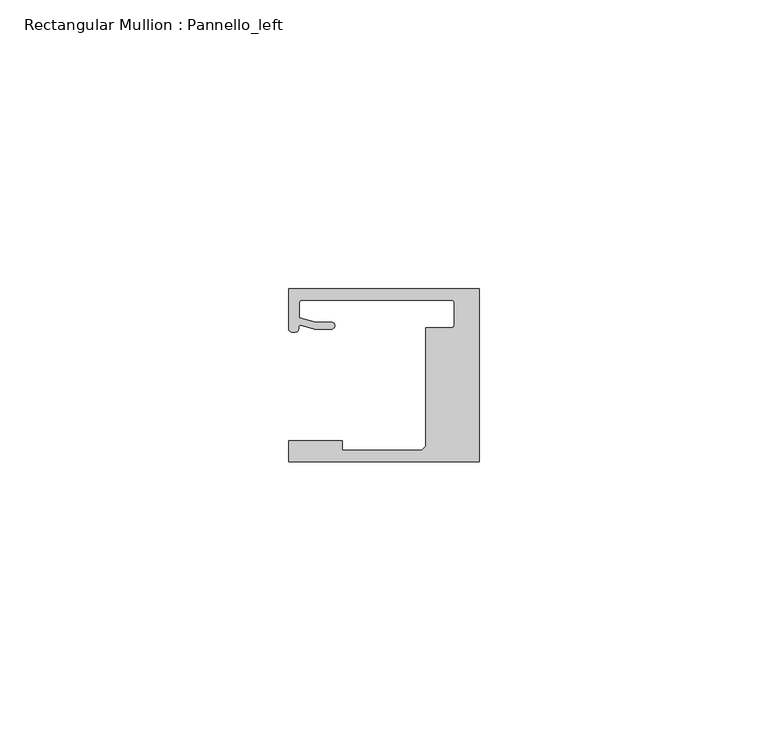
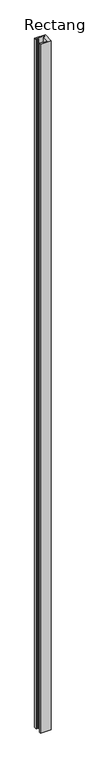
"""IFC4 building model written with IfcOpenShell, lengths in millimetres: member geometry, Rectangular Mullion : Pannello_left."""

from ifc_helpers import new_model, si_unit, frame, origin, place, context, project, spatial, polyline, circle_curve, source, transform, mapped, element, save
from ifc_brep_helpers import plane_surface, cylinder_surface, revolved_surface, extruded_surface, spline_curve, advanced_brep


def rectangular_mullion_pannello_left_b202d7d7(model_context):
    return source(origin(), model_context, "Body", "AdvancedBrep", [
        advanced_brep(
        [(-33.0, -15.0, 0.0), (0.0, -15.0, 0.0), (0.0, 15.0, 0.0), (-33.0000135, 15.0, 0.0), (-33.0000135, 8.0000472, 0.0), (-30.9223017, 8.6490241, 0.0), (-28.4999305, 7.9999523, 0.0), (-25.59998, 7.9999523, 0.0), (-25.59998, 9.1999523, 0.0), (-28.3419477, 9.1999523, 0.0), (-31.19998, 9.9657591, 0.0), (-31.19998, 12.50001, 0.0), (-30.69998, 13.00001, 0.0), (-4.7999726, 13.00001, 0.0), (-4.2999726, 12.50001, 0.0), (-4.2999726, 8.7500595, 0.0), (-4.7999726, 8.2500595, 0.0), (-9.2999726, 8.2500595, 0.0), (-9.2999726, -12.2999849, 0.0), (-10.0000103, -13.0000004, 0.0), (-23.700041, -13.0000004, 0.0), (-23.700041, -11.3000004, 0.0), (-33.0, -11.3000004, 0.0), (-33.0, -15.0, -2240.0), (-33.0, -11.3000004, -2240.0), (-23.700041, -11.3000004, -2240.0), (-23.700041, -13.0000004, -2240.0), (-10.0000103, -13.0000004, -2240.0), (-9.2999726, -12.2999849, -2240.0), (-9.2999726, 8.2500595, -2240.0), (-4.7999726, 8.2500595, -2240.0), (-4.2999726, 8.7500595, -2240.0), (-4.2999726, 12.50001, -2240.0), (-4.7999726, 13.00001, -2240.0), (-30.69998, 13.00001, -2240.0), (-31.19998, 12.50001, -2240.0), (-31.19998, 9.9657591, -2240.0), (-28.3419477, 9.1999523, -2240.0), (-25.59998, 9.1999523, -2240.0), (-25.59998, 7.9999523, -2240.0), (-28.4999305, 7.9999523, -2240.0), (-30.9223017, 8.6490241, -2240.0), (-33.0000135, 8.0000472, -2240.0), (-33.0000135, 15.0, -2240.0), (0.0, 15.0, -2240.0), (0.0, -15.0, -2240.0)],
        [
            (0, 1),
            (1, 2),
            (2, 3),
            (3, 4),
            (4, 5, spline_curve(3, [(-33.0000135, 8.0000472, 0.0), (-33.0000135, 7.457047519, 0.0), (-32.262327879, 7.456527435, 0.0), (-31.357433266, 7.563996614, 0.0), (-31.305645054, 7.690065204, 0.0), (-31.298563602, 8.366228555, 0.0), (-31.312054066, 8.717747958, 0.0), (-30.9223017, 8.6490241, 0.0)], [4, 2, 2, 4], [0.0, 0.0027053965905959043, 0.0058611956533709, 0.007702013405570312])),
            (5, 6),
            (6, 7),
            (7, 8, circle_curve(frame((-25.59998, 8.5999523, 0.0), z_axis=(0.0, 0.0, 1.0), x_axis=(0.0, 1.0, 0.0)), 0.6)),
            (8, 9),
            (9, 10),
            (10, 11),
            (11, 12, circle_curve(frame((-30.69998, 12.50001, 0.0), z_axis=(0.0, 0.0, -1.0), x_axis=(0.0, 1.0, 0.0)), 0.5)),
            (12, 13),
            (13, 14, circle_curve(frame((-4.7999726, 12.50001, 0.0), z_axis=(0.0, 0.0, -1.0), x_axis=(1.0, 0.0, 0.0)), 0.5)),
            (14, 15),
            (15, 16, circle_curve(frame((-4.7999726, 8.7500595, 0.0), z_axis=(0.0, 0.0, -1.0), x_axis=(0.0, -1.0, 0.0)), 0.5)),
            (16, 17),
            (17, 18),
            (18, 19),
            (19, 20),
            (20, 21),
            (21, 22),
            (22, 0),
            (23, 24),
            (24, 25),
            (25, 26),
            (26, 27),
            (27, 28),
            (28, 29),
            (29, 30),
            (30, 31, circle_curve(frame((-4.7999726, 8.7500595, -2240.0), z_axis=(0.0, 0.0, 1.0), x_axis=(0.0, -1.0, 0.0)), 0.5)),
            (31, 32),
            (32, 33, circle_curve(frame((-4.7999726, 12.50001, -2240.0), z_axis=(0.0, 0.0, 1.0), x_axis=(1.0, 0.0, 0.0)), 0.5)),
            (33, 34),
            (34, 35, circle_curve(frame((-30.69998, 12.50001, -2240.0), z_axis=(0.0, 0.0, 1.0), x_axis=(0.0, 1.0, 0.0)), 0.5)),
            (35, 36),
            (36, 37),
            (37, 38),
            (38, 39, circle_curve(frame((-25.59998, 8.5999523, -2240.0), z_axis=(0.0, 0.0, -1.0), x_axis=(0.0, 1.0, 0.0)), 0.6)),
            (39, 40),
            (40, 41),
            (41, 42, spline_curve(3, [(-30.9223017, 8.6490241, -2240.0), (-31.312054066, 8.717747958, -2240.0), (-31.298563602, 8.366228555, -2240.0), (-31.305645054, 7.690065204, -2240.0), (-31.357433266, 7.563996614, -2240.0), (-32.262327879, 7.456527435, -2240.0), (-33.0000135, 7.457047519, -2240.0), (-33.0000135, 8.0000472, -2240.0)], [4, 2, 2, 4], [0.0, 0.001840817752199412, 0.004996616814974408, 0.007702013405570312])),
            (42, 43),
            (43, 44),
            (44, 45),
            (45, 23),
            (0, 23),
            (45, 1),
            (44, 2),
            (43, 3),
            (42, 4),
            (41, 5),
            (40, 6),
            (39, 7),
            (38, 8),
            (37, 9),
            (36, 10),
            (35, 11),
            (34, 12),
            (33, 13),
            (32, 14),
            (31, 15),
            (30, 16),
            (29, 17),
            (28, 18),
            (27, 19),
            (26, 20),
            (25, 21),
            (24, 22),
        ],
        [
            plane_surface(frame((0.0, -36.2491502, 0.0), z_axis=(0.0, 0.0, 1.0), x_axis=(-1.0, 0.0, 0.0))),
            plane_surface(frame((0.0, -36.2491502, -2240.0), z_axis=(0.0, 0.0, -1.0), x_axis=(-1.0, 0.0, 0.0))),
            plane_surface(frame((-33.0, -15.0, 0.0), z_axis=(0.0, -1.0, 0.0), x_axis=(0.0, 0.0, -1.0))),
            plane_surface(frame((0.0, -15.0, 0.0), z_axis=(1.0, 0.0, 0.0), x_axis=(0.0, 0.0, -1.0))),
            plane_surface(frame((0.0, 15.0, 0.0), z_axis=(0.0, 1.0, 0.0), x_axis=(0.0, 0.0, -1.0))),
            plane_surface(frame((-33.0000135, 15.0, 0.0), z_axis=(-1.0, 0.0, 0.0), x_axis=(0.0, 0.0, -1.0))),
            extruded_surface(spline_curve(3, [(-33.0000135, 8.0000472, -2240.0), (-33.0000135, 7.457047519, -2240.0), (-32.262327879, 7.456527435, -2240.0), (-31.357433266, 7.563996614, -2240.0), (-31.305645054, 7.690065204, -2240.0), (-31.298563602, 8.366228555, -2240.0), (-31.312054066, 8.717747958, -2240.0), (-30.9223017, 8.6490241, -2240.0)], [4, 2, 2, 4], [0.0, 0.0027053965905959043, 0.0058611956533709, 0.007702013405570312]), (0.0, 0.0, 2240.0), 2240.0),
            plane_surface(frame((-30.9223017, 8.6490241, 0.0), z_axis=(-0.25881883200192934, -0.9659258833891746, 0.0), x_axis=(0.0, 0.0, -1.0))),
            plane_surface(frame((-28.4999305, 7.9999523, 0.0), z_axis=(0.0, -1.0, 0.0), x_axis=(0.0, 0.0, -1.0))),
            cylinder_surface(frame((-25.59998, 8.5999523, 0.0), z_axis=(0.0, 0.0, 1.0), x_axis=(0.0, 1.0, 0.0)), 0.6),
            plane_surface(frame((-25.59998, 9.1999523, 0.0), z_axis=(0.0, 1.0, 0.0), x_axis=(0.0, 0.0, -1.0))),
            plane_surface(frame((-28.3419477, 9.1999523, 0.0), z_axis=(0.25881883204288636, 0.9659258833782002, 0.0), x_axis=(0.0, 0.0, -1.0))),
            plane_surface(frame((-31.19998, 9.9657591, 0.0), z_axis=(1.0, 0.0, 0.0), x_axis=(0.0, 0.0, -1.0))),
            revolved_surface(polyline([(-30.69998, 13.00001, -2240.0), (-30.69998, 13.00001, 0.0)]), (-30.69998, 12.50001, 0.0), (0.0, 0.0, -1.0)),
            plane_surface(frame((-30.69998, 13.00001, 0.0), z_axis=(0.0, -1.0, 0.0), x_axis=(0.0, 0.0, -1.0))),
            revolved_surface(polyline([(-4.2999726, 12.50001, -2240.0), (-4.2999726, 12.50001, 0.0)]), (-4.7999726, 12.50001, 0.0), (0.0, 0.0, -1.0)),
            plane_surface(frame((-4.2999726, 12.50001, 0.0), z_axis=(-1.0, 0.0, 0.0), x_axis=(0.0, 0.0, -1.0))),
            revolved_surface(polyline([(-4.7999726, 8.2500595, -2240.0), (-4.7999726, 8.2500595, 0.0)]), (-4.7999726, 8.7500595, 0.0), (0.0, 0.0, -1.0)),
            plane_surface(frame((-4.7999726, 8.2500595, 0.0), z_axis=(0.0, 1.0, 0.0), x_axis=(0.0, 0.0, -1.0))),
            plane_surface(frame((-9.2999726, 8.2500595, 0.0), z_axis=(-1.0, 0.0, 0.0), x_axis=(0.0, 0.0, -1.0))),
            plane_surface(frame((-9.2999726, -12.2999849, 0.0), z_axis=(-0.7070955486277984, 0.7071180135668678, 0.0), x_axis=(0.0, 0.0, -1.0))),
            plane_surface(frame((-10.0000103, -13.0000004, 0.0), z_axis=(0.0, 1.0, 0.0), x_axis=(0.0, 0.0, -1.0))),
            plane_surface(frame((-23.700041, -13.0000004, 0.0), z_axis=(1.0, 0.0, 0.0), x_axis=(0.0, 0.0, -1.0))),
            plane_surface(frame((-23.700041, -11.3000004, 0.0), z_axis=(0.0, 1.0, 0.0), x_axis=(0.0, 0.0, -1.0))),
            plane_surface(frame((-33.0, -11.3000004, 0.0), z_axis=(-1.0, 0.0, 0.0), x_axis=(0.0, 0.0, -1.0))),
        ],
        [
            (0, [[1, 2, 3, 4, 5, 6, 7, 8, 9, 10, 11, 12, 13, 14, 15, 16, 17, 18, 19, 20, 21, 22, 23]]),
            (1, [[24, 25, 26, 27, 28, 29, 30, 31, 32, 33, 34, 35, 36, 37, 38, 39, 40, 41, 42, 43, 44, 45, 46]]),
            (2, [[-1, 47, -46, 48]]),
            (3, [[-2, -48, -45, 49]]),
            (4, [[-3, -49, -44, 50]]),
            (5, [[-4, -50, -43, 51]]),
            (6, [[-5, -51, -42, 52]]),
            (7, [[-6, -52, -41, 53]]),
            (8, [[-7, -53, -40, 54]]),
            (9, [[-8, -54, -39, 55]]),
            (10, [[-9, -55, -38, 56]]),
            (11, [[-10, -56, -37, 57]]),
            (12, [[-11, -57, -36, 58]]),
            (13, [[-12, -58, -35, 59]]),
            (14, [[-13, -59, -34, 60]]),
            (15, [[-14, -60, -33, 61]]),
            (16, [[-15, -61, -32, 62]]),
            (17, [[-16, -62, -31, 63]]),
            (18, [[-17, -63, -30, 64]]),
            (19, [[-18, -64, -29, 65]]),
            (20, [[-19, -65, -28, 66]]),
            (21, [[-20, -66, -27, 67]]),
            (22, [[-21, -67, -26, 68]]),
            (23, [[-22, -68, -25, 69]]),
            (24, [[-23, -69, -24, -47]]),
        ],
    ),
    ])


if __name__ == "__main__":
    model = new_model("IFC4")
    model_context = context("Model", 3, world=origin())
    ifc_project = project(units=[si_unit("LENGTHUNIT", "METRE", prefix="MILLI")], contexts=[model_context])
    site = spatial("IfcSite", under=ifc_project)
    building = spatial("IfcBuilding", under=site)
    placement = place(None, origin())
    rectangular_mullion_pannello_left_shape = rectangular_mullion_pannello_left_b202d7d7(model_context)
    element("IfcMember", 1, ObjectType="Rectangular Mullion : Pannello_left", at=placement, inside=building, context=model_context, shape_type="MappedRepresentation", body=[
        mapped(rectangular_mullion_pannello_left_shape, transform((0.0, 0.0, 0.0), x_axis=(1.0, 0.0, 0.0), y_axis=(0.0, 1.0, 0.0), z_axis=(0.0, 0.0, 1.0))),
    ])
    save(model, "model.ifc")

# Revit data of these elements
# Type "Rectangular Mullion : Pannello_left"
#   built-in parameter 1007322 = 0.0984252 (stored number, unit not read)
#   built-in parameter 1007320 = 0.0305117 (stored number, unit not read)
